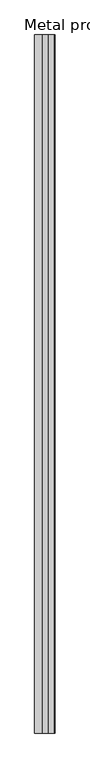
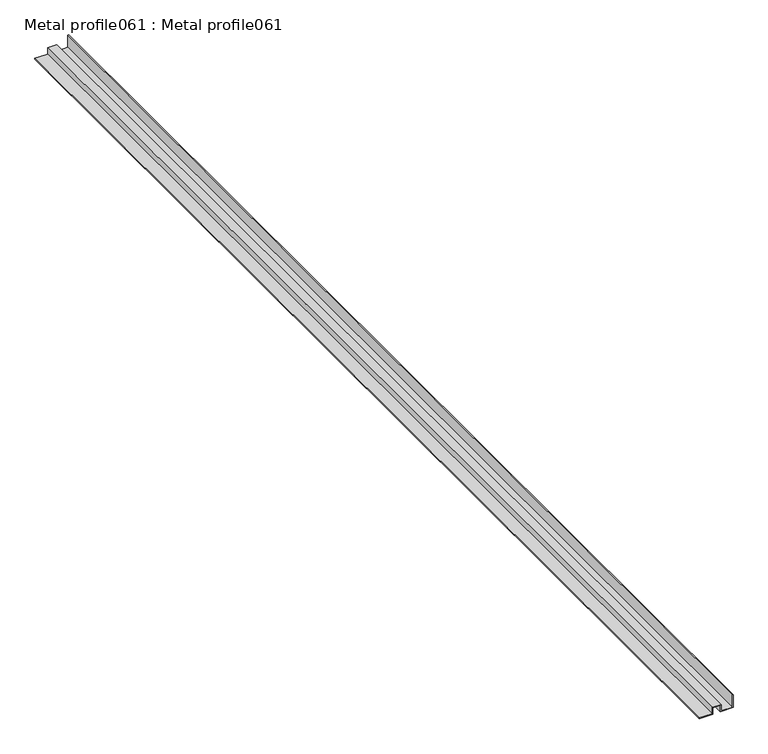
"""IFC4 building model written with IfcOpenShell, lengths in millimetres: proxy geometry, Metal profile061 : Metal profile061."""

import ifcopenshell
import ifcopenshell.guid

model = None  # the IFC model being written
_history = None  # IfcOwnerHistory: only IFC2X3 demands one
_inside = {}  # id of a spatial element -> (the spatial element, [elements in it])
_under = {}  # id of a project, library or spatial element -> (it, [spatial elements below it])
_declared = {}  # id of a project -> (the project, [libraries it declares])
_typed = {}  # id of a type object -> (the type object, [elements of that type])
_made_of = {}  # id of a material, layer set ... -> (it, [elements and type objects made of it])


def new_model(schema):
    """Start an empty IFC model of exactly this schema.

    Asked for "IFC4X3", IfcOpenShell would pick the latest addendum, in which some entities
    have other attributes; the version numbers below select the first issue.
    IFC2X3 requires an IfcOwnerHistory on every rooted entity: one is made here for all.
    """
    global model, _history
    if schema == "IFC4X3":
        model = ifcopenshell.file(schema_version=(4, 3, 0, 0))
    else:
        model = ifcopenshell.file(schema=schema)
    _inside.clear()
    _under.clear()
    _declared.clear()
    _typed.clear()
    _made_of.clear()
    _history = None
    if model.schema == "IFC2X3":
        org = make("IfcOrganization", Name="unknown")
        user = make(
            "IfcPersonAndOrganization",
            ThePerson=make("IfcPerson", FamilyName="unknown"),
            TheOrganization=org,
        )
        app = make(
            "IfcApplication",
            ApplicationDeveloper=org,
            Version="unknown",
            ApplicationFullName="unknown",
            ApplicationIdentifier="unknown",
        )
        _history = make(
            "IfcOwnerHistory",
            OwningUser=user,
            OwningApplication=app,
            ChangeAction="ADDED",
            CreationDate=0,
        )
    return model


def make(cls, **values):
    """One entity of the class cls with the attributes given. An attribute that is None is left unset."""
    return model.create_entity(
        cls, **{name: value for name, value in values.items() if value is not None}
    )


def rooted(cls, **values):
    """An entity with a GlobalId (a new one), such as an element, a storey or a relation."""
    return make(cls, GlobalId=ifcopenshell.guid.new(), OwnerHistory=_history, **values)


def si_unit(unit_type, name, prefix=None):
    """IfcSIUnit, for example si_unit("LENGTHUNIT", "METRE", prefix="MILLI")."""
    return make("IfcSIUnit", UnitType=unit_type, Prefix=prefix, Name=name)


def assignment(units):
    """IfcUnitAssignment: the units of a project."""
    return None if units is None else make("IfcUnitAssignment", Units=units)


def point(xyz):
    """IfcCartesianPoint."""
    return None if xyz is None else make("IfcCartesianPoint", Coordinates=xyz)


def direction(xyz):
    """IfcDirection."""
    return None if xyz is None else make("IfcDirection", DirectionRatios=xyz)


def frame(location, z_axis=None, x_axis=None):
    """IfcAxis2Placement3D, a coordinate frame: its origin and axes. An axis left out is left unset."""
    return make(
        "IfcAxis2Placement3D",
        Location=point(location),
        Axis=direction(z_axis),
        RefDirection=direction(x_axis),
    )


def origin():
    """The frame at (0, 0, 0) with its axes left unset."""
    return frame((0.0, 0.0, 0.0))


def place(relative_to, where):
    """IfcLocalPlacement: puts the frame where relative to a parent placement (None: the world)."""
    return make(
        "IfcLocalPlacement", PlacementRelTo=relative_to, RelativePlacement=where
    )


def context(
    kind, dimensions, precision=None, world=None, true_north=None, identifier=None
):
    """IfcGeometricRepresentationContext, for example the 3D "Model" context."""
    return make(
        "IfcGeometricRepresentationContext",
        ContextIdentifier=identifier,
        ContextType=kind,
        CoordinateSpaceDimension=dimensions,
        Precision=precision,
        WorldCoordinateSystem=world,
        TrueNorth=true_north,
    )


def project(units=None, contexts=None):
    """IfcProject with its units and contexts."""
    return rooted(
        "IfcProject",
        Name="project",
        RepresentationContexts=contexts,
        UnitsInContext=assignment(units),
    )


def spatial(cls, under=None, at=None, **own):
    """A site, building, storey or space (cls), placed at a placement, below another one or the project."""
    s = rooted(cls, ObjectPlacement=at, **own)
    if under is not None:
        _under.setdefault(under.id(), (under, []))[1].append(s)
    return s


def polyline(points):
    """IfcPolyline through the points."""
    return make("IfcPolyline", Points=[point(p) for p in points])


def outline(outer, holes=None, kind="AREA"):
    """IfcArbitraryClosedProfileDef: a profile drawn as a closed curve; with holes, ...WithVoids."""
    if holes is None:
        return make("IfcArbitraryClosedProfileDef", ProfileType=kind, OuterCurve=outer)
    return make(
        "IfcArbitraryProfileDefWithVoids",
        ProfileType=kind,
        OuterCurve=outer,
        InnerCurves=holes,
    )


def extrude(swept, where, along, depth):
    """IfcExtrudedAreaSolid: the profile swept, set in the frame where, extruded along a direction by depth."""
    return make(
        "IfcExtrudedAreaSolid",
        SweptArea=swept,
        Position=where,
        ExtrudedDirection=direction(along),
        Depth=depth,
    )


def shape(context_of_items, identifier, shape_type, items):
    """IfcShapeRepresentation: the items that make up one representation, for example the "Body"."""
    return make(
        "IfcShapeRepresentation",
        ContextOfItems=context_of_items,
        RepresentationIdentifier=identifier,
        RepresentationType=shape_type,
        Items=items,
    )


def source(mapping_origin, context_of_items, identifier, shape_type, items):
    """IfcRepresentationMap: a shape defined once, which mapped items show again and again."""
    return make(
        "IfcRepresentationMap",
        MappingOrigin=mapping_origin,
        MappedRepresentation=shape(context_of_items, identifier, shape_type, items),
    )


def transform(
    local_origin,
    x_axis=None,
    y_axis=None,
    z_axis=None,
    scale=None,
    scale2=None,
    scale3=None,
    uniform=True,
):
    """IfcCartesianTransformationOperator3D, or its non-uniform kind. x_axis, y_axis, z_axis: its Axis1, 2, 3."""
    if uniform:
        return make(
            "IfcCartesianTransformationOperator3D",
            Axis1=direction(x_axis),
            Axis2=direction(y_axis),
            LocalOrigin=point(local_origin),
            Scale=scale,
            Axis3=direction(z_axis),
        )
    return make(
        "IfcCartesianTransformationOperator3DnonUniform",
        Axis1=direction(x_axis),
        Axis2=direction(y_axis),
        LocalOrigin=point(local_origin),
        Scale=scale,
        Axis3=direction(z_axis),
        Scale2=scale2,
        Scale3=scale3,
    )


def mapped(mapping_source, mapping_target):
    """IfcMappedItem: shows the shape of a source again, moved by a transform."""
    return make(
        "IfcMappedItem", MappingSource=mapping_source, MappingTarget=mapping_target
    )


def made_of(thing, what):
    """Note that an element or type object is made of a material, layer set ...; save() writes the relation."""
    if what is not None:
        _made_of.setdefault(what.id(), (what, []))[1].append(thing)
    return thing


def element(
    cls,
    number,
    at=None,
    inside=None,
    cuts=None,
    type_object=None,
    material=None,
    context=None,
    identifier="Body",
    shape_type=None,
    held_by="IfcProductDefinitionShape",
    body=None,
    shapes=None,
    **own,
):
    """One element of the class cls, such as IfcWall. Its Tag is "e" and its number.

    at: its placement. inside: the storey or other place that contains it. cuts: it is an
    opening in that element (IfcRelVoidsElement). A single representation is given by context,
    identifier, shape_type and body (its items); several are given by shapes. held_by: the class
    of the entity that holds the representations. save() writes the other relations.
    """
    e = rooted(cls, Tag="e%d" % number, ObjectPlacement=at, **own)
    if body is not None:
        shapes = [shape(context, identifier, shape_type, body)]
    if shapes is not None:
        e.Representation = make(held_by, Representations=shapes)
    if inside is not None:
        _inside.setdefault(inside.id(), (inside, []))[1].append(e)
    if cuts is not None:
        rooted(
            "IfcRelVoidsElement", RelatingBuildingElement=cuts, RelatedOpeningElement=e
        )
    if type_object is not None:
        _typed.setdefault(type_object.id(), (type_object, []))[1].append(e)
    return made_of(e, material)


def aggregate(whole, parts):
    """IfcRelAggregates: a whole, such as a stair, and the parts it consists of."""
    return rooted("IfcRelAggregates", RelatingObject=whole, RelatedObjects=parts)


def save(model, path):
    """Write the relations noted so far, then the file.

    IfcRelAggregates (storeys below a building ...), IfcRelContainedInSpatialStructure (elements
    in a storey), IfcRelDefinesByType, IfcRelAssociatesMaterial and IfcRelDeclares: one each for
    every whole, place, type object, material and project.
    """
    for whole, parts in _under.values():
        aggregate(whole, parts)
    for where, things in _inside.values():
        rooted(
            "IfcRelContainedInSpatialStructure",
            RelatedElements=things,
            RelatingStructure=where,
        )
    for kind, things in _typed.values():
        rooted("IfcRelDefinesByType", RelatedObjects=things, RelatingType=kind)
    for what, things in _made_of.values():
        rooted("IfcRelAssociatesMaterial", RelatedObjects=things, RelatingMaterial=what)
    for by, libraries in _declared.values():
        rooted("IfcRelDeclares", RelatingContext=by, RelatedDefinitions=libraries)
    model.write(path)


def metal_profile061_metal_profile061_640eaa85(model_context):
    return source(origin(), model_context, "Body", "SweptSolid", [
        extrude(outline(polyline([(39543.8875708, -639.211476), (39567.6883323, -639.211476), (39567.6883323, -640.491476), (39545.1675708, -640.491476), (39545.1675708, -660.156476), (39556.5975708, -660.156476), (39556.5975708, -675.416476), (39545.1675708, -675.416476), (39545.1675708, -697.84966), (39543.8875708, -697.84966), (39543.8875708, -674.136476), (39555.3175708, -674.136476), (39555.3175708, -661.436476), (39543.8875708, -661.436476), (39543.8875708, -639.211476)])), frame((0.0, -1052.8906574, 0.0), z_axis=(0.0, 1.0, 0.0), x_axis=(0.0, 0.0, 1.0)), (0.0, 0.0, 1.0), 2000.0),
    ])


if __name__ == "__main__":
    model = new_model("IFC4")
    model_context = context("Model", 3, world=origin())
    ifc_project = project(units=[si_unit("LENGTHUNIT", "METRE", prefix="MILLI")], contexts=[model_context])
    site = spatial("IfcSite", under=ifc_project)
    building = spatial("IfcBuilding", under=site)
    placement = place(None, origin())
    metal_profile061_metal_profile061_shape = metal_profile061_metal_profile061_640eaa85(model_context)
    element("IfcBuildingElementProxy", 1, Name="Metal profile061 : Metal profile061", ObjectType="Metal profile061 : Metal profile061", at=placement, inside=building, context=model_context, shape_type="MappedRepresentation", body=[
        mapped(metal_profile061_metal_profile061_shape, transform((0.0, 0.0, 0.0), x_axis=(1.0, 0.0, 0.0), y_axis=(0.0, 1.0, 0.0), z_axis=(0.0, 0.0, 1.0))),
    ])
    save(model, "model.ifc")

# Revit data of these elements
# Type "Metal profile061 : Metal profile061"
#   NameOverride = "Metal profile061"
# Element 1 (IfcBuildingElementProxy, "Metal profile061 : Metal profile061")
#   Materials on its faces: "16 GA. COPPER SOFFIT DRIP SCREED"
# Materials
#   "16 GA. COPPER SOFFIT DRIP SCREED": class "Unassigned", colour RGB 255 217 0, transparency 0
